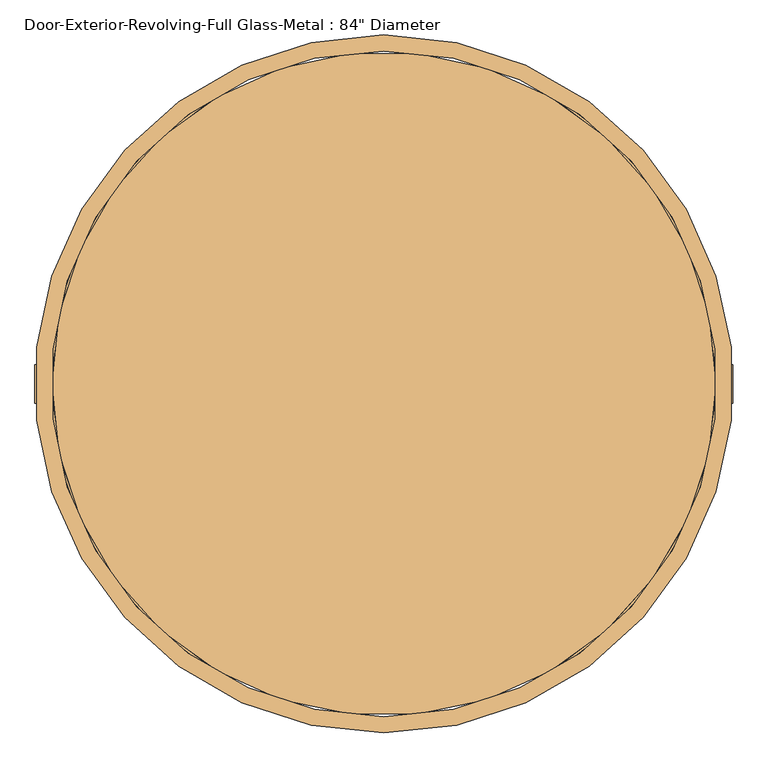
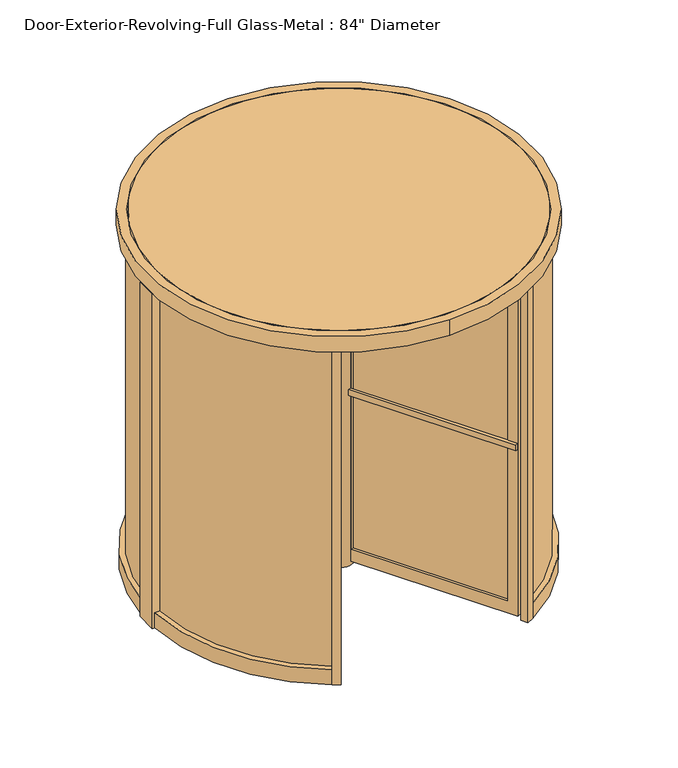
"""IFC4 building model written with IfcOpenShell, lengths in millimetres: door geometry."""

from ifc_helpers import new_model, si_unit, point, frame, frame_2d, origin, origin_with_axes, origin_2d, place, context, project, spatial, polyline, circle_curve, trimmed, segment, composite_curve, outline, extrude, source, transform, mapped, element, save
from ifc_brep_helpers import plane_surface, revolved_surface, advanced_brep


def door_f17faca2(model_context):
    return source(origin(), model_context, "Body", "SolidModel", [
        advanced_brep(
        [(44.45, -76.9896584, 25.4), (44.45, -76.9896584, 2219.325), (59.9152559, -65.6762674, 2219.325), (59.9152559, -65.6762674, 25.4), (26.9196881, -84.7262674, 25.4), (26.9196881, -84.7262674, 2219.325), (558.1772161, -1004.8912978, 25.4), (558.1772161, -1004.8912978, 2219.325), (29.5397161, -89.2642891, 2152.65), (524.8397161, -947.149054, 2152.65), (524.8397161, -947.149054, 106.3625), (29.5397161, -89.2642891, 106.3625), (591.1727839, -985.8412978, 2219.325), (591.1727839, -985.8412978, 25.4), (62.5352839, -70.2142891, 2152.65), (62.5352839, -70.2142891, 106.3625), (557.8352839, -928.099054, 106.3625), (557.8352839, -928.099054, 2152.65)],
        [
            (0, 1),
            (1, 2, circle_curve(frame((0.0, 0.0, 2219.325), z_axis=(0.0, 0.0, 1.0), x_axis=(0.4999999999999996, -0.8660254037844389, 0.0)), 88.9)),
            (2, 3),
            (3, 0, circle_curve(frame((0.0, 0.0, 25.4), z_axis=(0.0, 0.0, -1.0), x_axis=(0.4999999999999996, -0.8660254037844389, 0.0)), 88.9)),
            (0, 4, circle_curve(frame((0.0, 0.0, 25.4), z_axis=(0.0, 0.0, -1.0), x_axis=(0.4999999999999996, -0.8660254037844389, 0.0)), 88.9)),
            (4, 5),
            (5, 1, circle_curve(frame((0.0, 0.0, 2219.325), z_axis=(0.0, 0.0, 1.0), x_axis=(0.4999999999999996, -0.8660254037844389, 0.0)), 88.9)),
            (6, 7),
            (7, 5),
            (4, 6),
            (8, 9),
            (9, 10),
            (10, 11),
            (11, 8),
            (12, 13),
            (13, 3),
            (2, 12),
            (14, 15),
            (15, 16),
            (16, 17),
            (17, 14),
            (7, 12),
            (6, 13),
            (11, 15),
            (14, 8),
            (10, 16),
            (9, 17),
        ],
        [
            revolved_surface(polyline([(44.44999999999997, -76.98965839643662, 2219.325), (44.44999999999997, -76.98965839643662, 25.399999999999977)]), (0.0, 0.0, -344.4385455), (0.0, 0.0, 1.0)),
            plane_surface(frame((-3.7977839, -31.5220453, 2219.325), z_axis=(-0.8660254037844389, -0.4999999999999996, 0.0), x_axis=(0.0, 0.0, -1.0))),
            plane_surface(frame((29.1977839, -12.4720453, 2219.325), z_axis=(0.8660254037844389, 0.4999999999999996, 0.0), x_axis=(0.0, 0.0, 1.0))),
            plane_surface(frame((558.1772161, -1004.8912978, 2219.325), z_axis=(0.0, 0.0, 1.0), x_axis=(0.8660254037844384, 0.5000000000000004, 0.0))),
            plane_surface(frame((558.1772161, -1004.8912978, 25.4), z_axis=(0.5000000000000004, -0.8660254037844384, 0.0), x_axis=(0.8660254037844384, 0.5000000000000004, 0.0))),
            plane_surface(frame((-3.7977839, -31.5220453, 25.4), z_axis=(0.0, 0.0, -1.0), x_axis=(0.8660254037844389, 0.49999999999999956, 0.0))),
            plane_surface(frame((29.5397161, -89.2642891, 106.3625), z_axis=(0.49999999999999983, -0.8660254037844388, 0.0), x_axis=(0.8660254037844388, 0.49999999999999983, 0.0))),
            plane_surface(frame((524.8397161, -947.149054, 106.3625), z_axis=(0.0, 0.0, 1.0), x_axis=(0.8660254037844404, 0.49999999999999706, 0.0))),
            plane_surface(frame((524.8397161, -947.149054, 2152.65), z_axis=(-0.49999999999999706, 0.8660254037844404, 0.0), x_axis=(0.8660254037844404, 0.49999999999999706, 0.0))),
            plane_surface(frame((29.5397161, -89.2642891, 2152.65), z_axis=(0.0, 0.0, -1.0), x_axis=(0.8660254037844389, 0.49999999999999967, 0.0))),
        ],
        [
            (0, [[1, 2, 3, 4]]),
            (0, [[-1, 5, 6, 7]]),
            (1, [[8, 9, -6, 10], [11, 12, 13, 14]]),
            (2, [[15, 16, -3, 17], [18, 19, 20, 21]]),
            (3, [[22, -17, -2, -7, -9]]),
            (4, [[-8, 23, -15, -22]]),
            (5, [[-23, -10, -5, -4, -16]]),
            (6, [[-14, 24, -18, 25]]),
            (7, [[-13, 26, -19, -24]]),
            (8, [[-12, 27, -20, -26]]),
            (9, [[-11, -25, -21, -27]]),
        ],
    ),
        advanced_brep(
        [(-1149.35, -19.05, 2219.325), (-1149.35, -19.05, 25.4), (-86.834944, -19.05, 25.4), (-86.834944, -19.05, 2219.325), (-92.075, -19.05, 2152.65), (-92.075, -19.05, 106.3625), (-1082.675, -19.05, 106.3625), (-1082.675, -19.05, 2152.65), (-1149.35, 19.05, 25.4), (-1149.35, 19.05, 2219.325), (-86.834944, 19.05, 2219.325), (-86.834944, 19.05, 25.4), (-92.075, 19.05, 2152.65), (-1082.675, 19.05, 2152.65), (-1082.675, 19.05, 106.3625), (-92.075, 19.05, 106.3625)],
        [
            (0, 1),
            (1, 2),
            (2, 3),
            (3, 0),
            (4, 5),
            (5, 6),
            (6, 7),
            (7, 4),
            (8, 9),
            (9, 10),
            (10, 11),
            (11, 8),
            (12, 13),
            (13, 14),
            (14, 15),
            (15, 12),
            (9, 0),
            (3, 10, circle_curve(frame((0.0, 0.0, 2219.325), z_axis=(0.0, 0.0, -1.0), x_axis=(0.4999999999999996, -0.8660254037844389, 0.0)), 88.9)),
            (8, 1),
            (11, 2, circle_curve(frame((0.0, 0.0, 25.4), z_axis=(0.0, 0.0, 1.0), x_axis=(0.4999999999999996, -0.8660254037844389, 0.0)), 88.9)),
            (4, 12),
            (15, 5),
            (14, 6),
            (13, 7),
        ],
        [
            plane_surface(frame((-1149.35, -19.05, 2219.325), z_axis=(0.0, -1.0, 0.0), x_axis=(-1.0, 0.0, 0.0))),
            plane_surface(frame((-1149.35, 19.05, 2219.325), z_axis=(0.0, 1.0, 0.0), x_axis=(1.0, 0.0, 0.0))),
            plane_surface(frame((-25.4, -19.05, 2219.325), z_axis=(0.0, 0.0, 1.0), x_axis=(0.0, 1.0, 0.0))),
            plane_surface(frame((-1149.35, -19.05, 2219.325), z_axis=(-1.0, 0.0, 0.0), x_axis=(0.0, 1.0, 0.0))),
            plane_surface(frame((-1149.35, -19.05, 25.4), z_axis=(0.0, 0.0, -1.0), x_axis=(0.0, 1.0, 0.0))),
            plane_surface(frame((-92.075, -19.05, 2152.65), z_axis=(-1.0, 0.0, 0.0), x_axis=(0.0, 1.0, 0.0))),
            plane_surface(frame((-92.075, -19.05, 106.3625), z_axis=(0.0, 0.0, 1.0), x_axis=(0.0, 1.0, 0.0))),
            plane_surface(frame((-1082.675, -19.05, 106.3625), z_axis=(1.0, 0.0, 0.0), x_axis=(0.0, 1.0, 0.0))),
            plane_surface(frame((-1082.675, -19.05, 2152.65), z_axis=(0.0, 0.0, -1.0), x_axis=(0.0, 1.0, 0.0))),
            revolved_surface(polyline([(44.44999999999997, -76.98965839643662, 2219.325), (44.44999999999997, -76.98965839643662, 25.399999999999977)]), (0.0, 0.0, -344.4385455), (0.0, 0.0, 1.0)),
        ],
        [
            (0, [[1, 2, 3, 4], [5, 6, 7, 8]]),
            (1, [[9, 10, 11, 12], [13, 14, 15, 16]]),
            (2, [[17, -4, 18, -10]]),
            (3, [[-1, -17, -9, 19]]),
            (4, [[-19, -12, 20, -2]]),
            (5, [[-5, 21, -16, 22]]),
            (6, [[-6, -22, -15, 23]]),
            (7, [[-7, -23, -14, 24]]),
            (8, [[-8, -24, -13, -21]]),
            (9, [[-3, -20, -11, -18]]),
        ],
    ),
        advanced_brep(
        [(591.1727839, 985.8412978, 25.4), (591.1727839, 985.8412978, 2219.325), (59.9152559, 65.6762674, 2219.325), (59.9152559, 65.6762674, 25.4), (62.5352839, 70.2142891, 2152.65), (557.8352839, 928.099054, 2152.65), (557.8352839, 928.099054, 106.3625), (62.5352839, 70.2142891, 106.3625), (558.1772161, 1004.8912978, 2219.325), (558.1772161, 1004.8912978, 25.4), (26.9196881, 84.7262674, 25.4), (26.9196881, 84.7262674, 2219.325), (29.5397161, 89.2642891, 2152.65), (29.5397161, 89.2642891, 106.3625), (524.8397161, 947.149054, 106.3625), (524.8397161, 947.149054, 2152.65)],
        [
            (0, 1),
            (1, 2),
            (2, 3),
            (3, 0),
            (4, 5),
            (5, 6),
            (6, 7),
            (7, 4),
            (8, 9),
            (9, 10),
            (10, 11),
            (11, 8),
            (12, 13),
            (13, 14),
            (14, 15),
            (15, 12),
            (1, 8),
            (11, 2, circle_curve(frame((0.0, 0.0, 2219.325), z_axis=(0.0, 0.0, -1.0), x_axis=(0.4999999999999996, -0.8660254037844389, 0.0)), 88.9)),
            (0, 9),
            (3, 10, circle_curve(frame((0.0, 0.0, 25.4), z_axis=(0.0, 0.0, 1.0), x_axis=(0.4999999999999996, -0.8660254037844389, 0.0)), 88.9)),
            (7, 13),
            (12, 4),
            (6, 14),
            (5, 15),
        ],
        [
            plane_surface(frame((29.1977839, 12.4720453, 2219.325), z_axis=(0.866025403784439, -0.4999999999999995, 0.0), x_axis=(0.0, 0.0, -1.0))),
            plane_surface(frame((-3.7977839, 31.5220453, 2219.325), z_axis=(-0.866025403784439, 0.4999999999999995, 0.0), x_axis=(0.0, 0.0, 1.0))),
            plane_surface(frame((591.1727839, 985.8412978, 2219.325), z_axis=(0.0, 0.0, 1.0), x_axis=(-0.8660254037844384, 0.5000000000000004, 0.0))),
            plane_surface(frame((591.1727839, 985.8412978, 25.4), z_axis=(0.5000000000000004, 0.8660254037844384, 0.0), x_axis=(-0.8660254037844384, 0.5000000000000004, 0.0))),
            plane_surface(frame((29.1977839, 12.4720453, 25.4), z_axis=(0.0, 0.0, -1.0), x_axis=(-0.866025403784439, 0.49999999999999944, 0.0))),
            plane_surface(frame((62.5352839, 70.2142891, 106.3625), z_axis=(0.49999999999999967, 0.8660254037844388, 0.0), x_axis=(-0.8660254037844388, 0.49999999999999967, 0.0))),
            plane_surface(frame((557.8352839, 928.099054, 106.3625), z_axis=(0.0, 0.0, 1.0), x_axis=(-0.8660254037844384, 0.5000000000000004, 0.0))),
            plane_surface(frame((557.8352839, 928.099054, 2152.65), z_axis=(-0.5000000000000004, -0.8660254037844384, 0.0), x_axis=(-0.8660254037844384, 0.5000000000000004, 0.0))),
            plane_surface(frame((62.5352839, 70.2142891, 2152.65), z_axis=(0.0, 0.0, -1.0), x_axis=(-0.866025403784439, 0.49999999999999944, 0.0))),
            revolved_surface(polyline([(44.44999999999997, -76.98965839643662, 2219.325), (44.44999999999997, -76.98965839643662, 25.399999999999977)]), (0.0, 0.0, -344.4385455), (0.0, 0.0, 1.0)),
        ],
        [
            (0, [[1, 2, 3, 4], [5, 6, 7, 8]]),
            (1, [[9, 10, 11, 12], [13, 14, 15, 16]]),
            (2, [[17, -12, 18, -2]]),
            (3, [[-1, 19, -9, -17]]),
            (4, [[-19, -4, 20, -10]]),
            (5, [[-8, 21, -13, 22]]),
            (6, [[-7, 23, -14, -21]]),
            (7, [[-6, 24, -15, -23]]),
            (8, [[-5, -22, -16, -24]]),
            (9, [[-3, -18, -11, -20]]),
        ],
    ),
        extrude(outline(composite_curve([segment(polyline([(-615.7921907, 989.2164973), (-638.1275667, 1031.4059972)]), True, "CONTINUOUS"), segment(trimmed(circle_curve(origin_2d(), 1212.85), [point((-638.1275667, 1031.4059972))], [point((-595.6078601, 1056.530359))], False, "CARTESIAN"), True, "CONTINUOUS"), segment(polyline([(-595.6078601, 1056.530359), (-573.2795251, 1014.4456056)]), True, "CONTINUOUS"), segment(trimmed(circle_curve(origin_2d(), 1165.225), [point((-573.2795251, 1014.4456056))], [point((-615.7921907, 989.2164973))], True, "CARTESIAN"), True, "CONTINUOUS")], self_intersect=False)), origin_with_axes(), (0.0, 0.0, 1.0), 2244.725),
        extrude(outline(composite_curve([segment(polyline([(638.2334006, 1031.6059079), (615.7921907, 989.2164973)]), True, "CONTINUOUS"), segment(trimmed(circle_curve(origin_2d(), 1165.225), [point((615.7921907, 989.2164973))], [point((573.2795251, 1014.4456056))], True, "CARTESIAN"), True, "CONTINUOUS"), segment(polyline([(573.2795251, 1014.4456056), (595.7136707, 1056.7297882)]), True, "CONTINUOUS"), segment(trimmed(circle_curve(origin_2d(), 1213.0756872), [point((595.7136707, 1056.7297882))], [point((638.2334006, 1031.6059079))], False, "CARTESIAN"), True, "CONTINUOUS")], self_intersect=False)), origin_with_axes(), (0.0, 0.0, 1.0), 2244.725),
        extrude(outline(composite_curve([segment(trimmed(circle_curve(origin_2d(), 1165.225), [point((-615.7921907, -989.2164973))], [point((-573.2795251, -1014.4456056))], True, "CARTESIAN"), True, "CONTINUOUS"), segment(polyline([(-573.2795251, -1014.4456056), (-595.6078601, -1052.8850325)]), True, "CONTINUOUS"), segment(trimmed(circle_curve(frame_2d((0.0, 179.0003095)), 1368.3165638), [point((-595.6078601, -1052.8850325))], [point((-638.1275667, -1031.4059972))], False, "CARTESIAN"), True, "CONTINUOUS"), segment(polyline([(-638.1275667, -1031.4059972), (-615.7921907, -989.2164973)]), True, "CONTINUOUS")], self_intersect=False)), origin_with_axes(), (0.0, 0.0, 1.0), 2244.725),
        extrude(outline(composite_curve([segment(trimmed(circle_curve(frame_2d((0.0, 179.0003498)), 1368.3165995), [point((638.1275667, -1031.4059972))], [point((595.6078689, -1052.8850275))], False, "CARTESIAN"), True, "CONTINUOUS"), segment(polyline([(595.6078689, -1052.8850275), (573.2795251, -1014.4456056)]), True, "CONTINUOUS"), segment(trimmed(circle_curve(origin_2d(), 1165.225), [point((573.2795251, -1014.4456056))], [point((615.7921907, -989.2164973))], True, "CARTESIAN"), True, "CONTINUOUS"), segment(polyline([(615.7921907, -989.2164973), (638.1275667, -1031.4059972)]), True, "CONTINUOUS")], self_intersect=False)), origin_with_axes(), (0.0, 0.0, 1.0), 2244.725),
        extrude(outline(composite_curve([segment(polyline([(-1171.2208243, 67.46875), (-1177.5812382, 67.46875)]), True, "CONTINUOUS"), segment(trimmed(circle_curve(origin_2d(), 1179.5124437), [point((-1177.5812382, 67.46875))], [point((-622.9714922, 1001.5768191))], False, "CARTESIAN"), True, "CONTINUOUS"), segment(polyline([(-622.9714922, 1001.5768191), (-619.7807004, 996.0833975)]), True, "CONTINUOUS"), segment(trimmed(circle_curve(origin_2d(), 1173.1625), [point((-619.7807004, 996.0833975))], [point((-1171.2208243, 67.46875))], True, "CARTESIAN"), True, "CONTINUOUS")], self_intersect=False)), frame((0.0, 0.0, 101.6), z_axis=(0.0, 0.0, 1.0), x_axis=(1.0, 0.0, 0.0)), (0.0, 0.0, 1.0), 2143.125),
        extrude(outline(composite_curve([segment(trimmed(circle_curve(origin_2d(), 1173.1625), [point((1171.2208243, 67.46875))], [point((619.7807004, 996.0833975))], True, "CARTESIAN"), True, "CONTINUOUS"), segment(polyline([(619.7807004, 996.0833975), (622.9714922, 1001.5768191)]), True, "CONTINUOUS"), segment(trimmed(circle_curve(origin_2d(), 1179.5124437), [point((622.9714922, 1001.5768191))], [point((1177.5812382, 67.46875))], False, "CARTESIAN"), True, "CONTINUOUS"), segment(polyline([(1177.5812382, 67.46875), (1171.2208243, 67.46875)]), True, "CONTINUOUS")], self_intersect=False)), frame((0.0, 0.0, 101.6), z_axis=(0.0, 0.0, 1.0), x_axis=(1.0, 0.0, 0.0)), (0.0, 0.0, 1.0), 2143.125),
        extrude(outline(composite_curve([segment(trimmed(circle_curve(origin_2d(), 1173.1625), [point((-1171.2208243, -67.46875))], [point((-619.7807004, -996.0833975))], True, "CARTESIAN"), True, "CONTINUOUS"), segment(polyline([(-619.7807004, -996.0833975), (-622.9714922, -1001.5768191)]), True, "CONTINUOUS"), segment(trimmed(circle_curve(origin_2d(), 1179.5124437), [point((-622.9714922, -1001.5768191))], [point((-1177.5812382, -67.46875))], False, "CARTESIAN"), True, "CONTINUOUS"), segment(polyline([(-1177.5812382, -67.46875), (-1171.2208243, -67.46875)]), True, "CONTINUOUS")], self_intersect=False)), frame((0.0, 0.0, 101.6), z_axis=(0.0, 0.0, 1.0), x_axis=(1.0, 0.0, 0.0)), (0.0, 0.0, 1.0), 2143.125),
        extrude(outline(composite_curve([segment(polyline([(1171.2208243, -67.46875), (1177.5812382, -67.46875)]), True, "CONTINUOUS"), segment(trimmed(circle_curve(origin_2d(), 1179.5124437), [point((1177.5812382, -67.46875))], [point((622.9714922, -1001.5768191))], False, "CARTESIAN"), True, "CONTINUOUS"), segment(polyline([(622.9714922, -1001.5768191), (619.7807004, -996.0833975)]), True, "CONTINUOUS"), segment(trimmed(circle_curve(origin_2d(), 1173.1625), [point((619.7807004, -996.0833975))], [point((1171.2208243, -67.46875))], True, "CARTESIAN"), True, "CONTINUOUS")], self_intersect=False)), frame((0.0, 0.0, 101.6), z_axis=(0.0, 0.0, 1.0), x_axis=(1.0, 0.0, 0.0)), (0.0, 0.0, 1.0), 2143.125),
        extrude(outline(composite_curve([segment(trimmed(circle_curve(origin_2d(), 1225.55), [point((0.0, -1225.55))], [point((0.0, 1225.55))], False, "CARTESIAN"), True, "CONTINUOUS"), segment(trimmed(circle_curve(origin_2d(), 1225.55), [point((0.0, 1225.55))], [point((0.0, -1225.55))], False, "CARTESIAN"), True, "CONTINUOUS")], self_intersect=False), holes=[composite_curve([segment(trimmed(circle_curve(origin_2d(), 1168.4), [point((0.0, 1168.4))], [point((0.0, -1168.4))], True, "CARTESIAN"), True, "CONTINUOUS"), segment(trimmed(circle_curve(origin_2d(), 1168.4), [point((0.0, -1168.4))], [point((0.0, 1168.4))], True, "CARTESIAN"), True, "CONTINUOUS")], self_intersect=False)]), frame((0.0, 0.0, 2244.725), z_axis=(0.0, 0.0, 1.0), x_axis=(1.0, 0.0, 0.0)), (0.0, 0.0, 1.0), 101.6),
        extrude(outline(composite_curve([segment(trimmed(circle_curve(origin_2d(), 1165.225), [point((-1165.225, 0.0))], [point((1165.225, 0.0))], False, "CARTESIAN"), True, "CONTINUOUS"), segment(trimmed(circle_curve(origin_2d(), 1165.225), [point((1165.225, 0.0))], [point((-1165.225, 0.0))], False, "CARTESIAN"), True, "CONTINUOUS")], self_intersect=False)), frame((0.0, 0.0, 2244.725), z_axis=(0.0, 0.0, 1.0), x_axis=(1.0, 0.0, 0.0)), (0.0, 0.0, 1.0), 101.6),
        extrude(outline(composite_curve([segment(trimmed(circle_curve(origin_2d(), 88.9), [point((-88.9, 0.0))], [point((88.9, 0.0))], False, "CARTESIAN"), True, "CONTINUOUS"), segment(trimmed(circle_curve(origin_2d(), 88.9), [point((88.9, 0.0))], [point((-88.9, 0.0))], False, "CARTESIAN"), True, "CONTINUOUS")], self_intersect=False)), origin_with_axes(), (0.0, 0.0, 1.0), 2244.725),
        extrude(outline(composite_curve([segment(polyline([(-615.7921907, -989.2164973), (-638.1275667, -1031.4059972)]), True, "CONTINUOUS"), segment(trimmed(circle_curve(origin_2d(), 1212.85), [point((-638.1275667, -1031.4059972))], [point((-1210.971961, -67.46875))], False, "CARTESIAN"), True, "CONTINUOUS"), segment(polyline([(-1210.971961, -67.46875), (-1163.2700754, -67.46875)]), True, "CONTINUOUS"), segment(trimmed(circle_curve(origin_2d(), 1165.225), [point((-1163.2700754, -67.46875))], [point((-615.7921907, -989.2164973))], True, "CARTESIAN"), True, "CONTINUOUS")], self_intersect=False)), origin_with_axes(), (0.0, 0.0, 1.0), 101.6),
        extrude(outline(composite_curve([segment(polyline([(638.1275667, -1031.4059972), (615.7921907, -989.2164973)]), True, "CONTINUOUS"), segment(trimmed(circle_curve(origin_2d(), 1165.225), [point((615.7921907, -989.2164973))], [point((1163.2700754, -67.46875))], True, "CARTESIAN"), True, "CONTINUOUS"), segment(polyline([(1163.2700754, -67.46875), (1210.971961, -67.46875)]), True, "CONTINUOUS"), segment(trimmed(circle_curve(origin_2d(), 1212.85), [point((1210.971961, -67.46875))], [point((638.1275667, -1031.4059972))], False, "CARTESIAN"), True, "CONTINUOUS")], self_intersect=False)), origin_with_axes(), (0.0, 0.0, 1.0), 101.6),
        extrude(outline(composite_curve([segment(polyline([(1210.971961, 67.46875), (1163.2700754, 67.46875)]), True, "CONTINUOUS"), segment(trimmed(circle_curve(origin_2d(), 1165.225), [point((1163.2700754, 67.46875))], [point((615.7921907, 989.2164973))], True, "CARTESIAN"), True, "CONTINUOUS"), segment(polyline([(615.7921907, 989.2164973), (638.1275667, 1031.4059972)]), True, "CONTINUOUS"), segment(trimmed(circle_curve(origin_2d(), 1212.85), [point((638.1275667, 1031.4059972))], [point((1210.971961, 67.46875))], False, "CARTESIAN"), True, "CONTINUOUS")], self_intersect=False)), origin_with_axes(), (0.0, 0.0, 1.0), 101.6),
        extrude(outline(composite_curve([segment(polyline([(-638.1275667, 1031.4059972), (-615.7921907, 989.2164973)]), True, "CONTINUOUS"), segment(trimmed(circle_curve(origin_2d(), 1165.225), [point((-615.7921907, 989.2164973))], [point((-1163.2700754, 67.46875))], True, "CARTESIAN"), True, "CONTINUOUS"), segment(polyline([(-1163.2700754, 67.46875), (-1210.971961, 67.46875)]), True, "CONTINUOUS"), segment(trimmed(circle_curve(origin_2d(), 1212.85), [point((-1210.971961, 67.46875))], [point((-638.1275667, 1031.4059972))], False, "CARTESIAN"), True, "CONTINUOUS")], self_intersect=False)), origin_with_axes(), (0.0, 0.0, 1.0), 101.6),
        extrude(outline(polyline([(-1168.4, 67.46875), (-1168.4, -67.46875), (-1225.55, -67.46875), (-1225.55, 67.46875), (-1168.4, 67.46875)])), origin_with_axes(), (0.0, 0.0, 1.0), 2244.725),
        extrude(outline(polyline([(1225.55, 67.46875), (1225.55, -67.46875), (1168.4, -67.46875), (1168.4, 67.46875), (1225.55, 67.46875)])), origin_with_axes(), (0.0, 0.0, 1.0), 2244.725),
        extrude(outline(polyline([(538.5878693, -939.211554), (43.2878693, -81.3267891), (48.7871307, -78.1517891), (544.0871307, -936.036554), (538.5878693, -939.211554)])), frame((0.0, 0.0, 106.3625), z_axis=(0.0, 0.0, 1.0), x_axis=(1.0, 0.0, 0.0)), (0.0, 0.0, 1.0), 2046.2875),
        extrude(outline(polyline([(544.0871307, 936.036554), (48.7871307, 78.1517891), (43.2878693, 81.3267891), (538.5878693, 939.211554), (544.0871307, 936.036554)])), frame((0.0, 0.0, 106.3625), z_axis=(0.0, 0.0, 1.0), x_axis=(1.0, 0.0, 0.0)), (0.0, 0.0, 1.0), 2046.2875),
        extrude(outline(polyline([(-92.075, -3.175), (-1082.675, -3.175), (-1082.675, 3.175), (-92.075, 3.175), (-92.075, -3.175)])), frame((0.0, 0.0, 106.3625), z_axis=(0.0, 0.0, 1.0), x_axis=(1.0, 0.0, 0.0)), (0.0, 0.0, 1.0), 2046.2875),
        extrude(outline(composite_curve([segment(polyline([(-1149.35, 19.05), (-1149.35, 38.1), (-80.3218526, 38.1)]), True, "CONTINUOUS"), segment(trimmed(circle_curve(origin_2d(), 88.9), [point((-80.3218526, 38.1))], [point((-86.834944, 19.05))], True, "CARTESIAN"), True, "CONTINUOUS"), segment(polyline([(-86.834944, 19.05), (-1149.35, 19.05)]), True, "CONTINUOUS")], self_intersect=False)), frame((0.0, 0.0, 1149.35), z_axis=(0.0, 0.0, 1.0), x_axis=(1.0, 0.0, 0.0)), (0.0, 0.0, 1.0), 38.1),
        extrude(outline(composite_curve([segment(polyline([(558.1772161, -1004.8912978), (541.6794321, -1014.4162978), (7.1653584, -88.6107648)]), True, "CONTINUOUS"), segment(trimmed(circle_curve(origin_2d(), 88.9), [point((7.1653584, -88.6107648))], [point((26.9196881, -84.7262674))], True, "CARTESIAN"), True, "CONTINUOUS"), segment(polyline([(26.9196881, -84.7262674), (558.1772161, -1004.8912978)]), True, "CONTINUOUS")], self_intersect=False)), frame((0.0, 0.0, 1149.35), z_axis=(0.0, 0.0, 1.0), x_axis=(1.0, 0.0, 0.0)), (0.0, 0.0, 1.0), 38.1),
        extrude(outline(composite_curve([segment(polyline([(591.1727839, 985.8412978), (607.6705679, 976.3162978), (73.1564942, 50.5107648)]), True, "CONTINUOUS"), segment(trimmed(circle_curve(origin_2d(), 88.9), [point((73.1564942, 50.5107648))], [point((59.9152559, 65.6762674))], True, "CARTESIAN"), True, "CONTINUOUS"), segment(polyline([(59.9152559, 65.6762674), (591.1727839, 985.8412978)]), True, "CONTINUOUS")], self_intersect=False)), frame((0.0, 0.0, 1149.35), z_axis=(0.0, 0.0, 1.0), x_axis=(1.0, 0.0, 0.0)), (0.0, 0.0, 1.0), 38.1),
    ])


if __name__ == "__main__":
    model = new_model("IFC4")
    model_context = context("Model", 3, world=origin())
    ifc_project = project(units=[si_unit("LENGTHUNIT", "METRE", prefix="MILLI")], contexts=[model_context])
    site = spatial("IfcSite", under=ifc_project)
    building = spatial("IfcBuilding", under=site)
    placement = place(None, origin())
    door_shape = door_f17faca2(model_context)
    element("IfcDoor", 1, ObjectType="Door-Exterior-Revolving-Full Glass-Metal : 84\" Diameter", at=placement, inside=building, context=model_context, shape_type="MappedRepresentation", body=[
        mapped(door_shape, transform((0.0, 0.0, 0.0), x_axis=(1.0, 0.0, 0.0), y_axis=(0.0, 1.0, 0.0), z_axis=(0.0, 0.0, 1.0))),
    ])
    save(model, "model.ifc")

# Revit data of these elements
# Type "Door-Exterior-Revolving-Full Glass-Metal : 84\" Diameter"
#   Type Mark = "35"
#   Assembly Code = "B2030300"
#   Analytic Construction = "Metal frame, double glass door"
#   Width = 8' - 0"
#   Thermal Resistance (R) = 1.3794 (h·ft²·°F)/BTU
#   Rough Width = 8' - 0 1/2"
#   Rough Height = 7' - 8 3/8"
#   Push Bar Height = 3' - 10"
#   Panel Width = 3' - 8 1/4"
#   Outside Diameter = 8' - 0 1/2"
#   Inside Radius = 3' - 9 7/8"
#   Inside Diameter = 7' - 7 3/4"
#   Height = 7' - 8"
#   Heat Transfer Coefficient (U) = 0.7250 BTU/(h·ft²·°F)
#   Glazing Radius = 3' - 10 3/16"
#   Door Opening Width = 3' - 9 1/8"
#   Function = 1
#   Push Bar Material = Aluminum
#   Panel Material = Aluminum
#   Glazing = Glass
#   Frame Material = Aluminum
#   Wall Closure = (empty or 0)
#   Visual Light Transmittance = 0
#   Solar Heat Gain Coefficient = 0
# Element 1 (IfcDoor, "Door-Exterior-Revolving-Full Glass-Metal : 84\" Diameter")
#   Materials on its faces: "Aluminum", "Glass"
# Materials
#   "Aluminum": class "Metal", colour RGB 120 120 120, transparency 0, Description = "Aluminum 6061", Cost = 0
#   "Glass": class "Unassigned", colour RGB 0 128 192, transparency 0.75, Description = "Glass"
